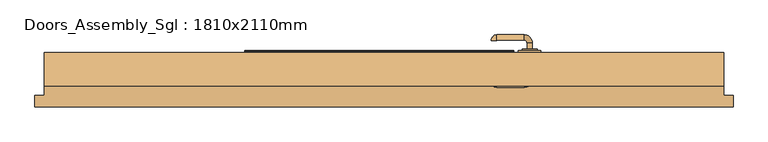
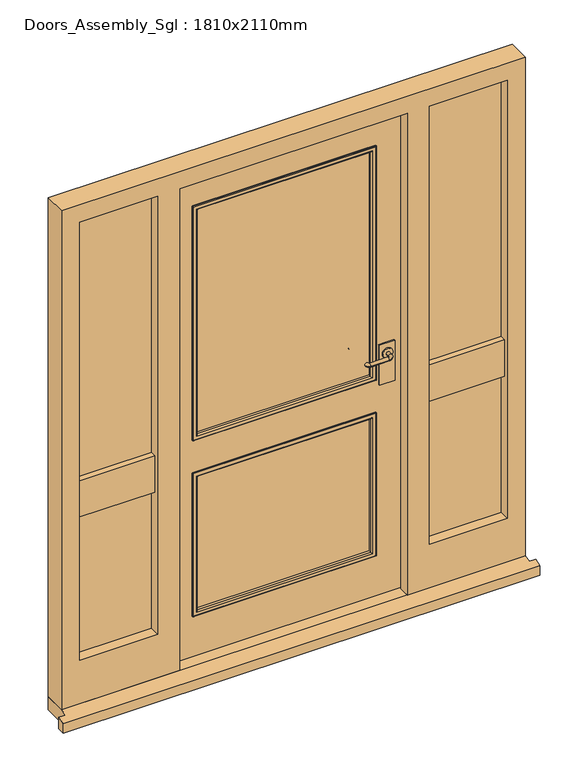
"""IFC4 building model written with IfcOpenShell, lengths in millimetres: door geometry, Doors_Assembly_Sgl : 1810x2110mm."""

from ifc_helpers import new_model, si_unit, point, frame, frame_2d, origin, place, context, project, spatial, polyline, circle_curve, ellipse_curve, trimmed, segment, composite_curve, outline, extrude, faceted_brep, source, transform, mapped, element, save
from ifc_brep_helpers import plane_surface, cylinder_surface, revolved_surface, advanced_brep


def doors_assembly_sgl_1810x2110mm_cdd653b2(model_context):
    return source(origin(), model_context, "Body", "SolidModel", [
        extrude(outline(composite_curve([segment(trimmed(circle_curve(frame_2d((1050.0, 680.0)), 20.0), [point((1050.0, 700.0))], [point((1050.0, 660.0))], False, "CARTESIAN"), True, "CONTINUOUS"), segment(trimmed(circle_curve(frame_2d((1050.0, 680.0)), 20.0), [point((1050.0, 660.0))], [point((1050.0, 700.0))], False, "CARTESIAN"), True, "CONTINUOUS")], self_intersect=False)), frame((0.0, -42.25, 0.0), z_axis=(0.0, 1.0, 0.0), x_axis=(0.0, 0.0, 1.0)), (0.0, 0.0, 1.0), 4.5929895),
        advanced_brep(
        [(673.0, -37.6570105, 1050.0), (687.0, -37.6570105, 1050.0), (687.0, -22.25, 1050.0), (673.0, -22.25, 1050.0), (665.0, -0.25, 1050.0), (665.0, -14.25, 1050.0), (593.0, -0.25, 1050.0), (593.0, -14.25, 1050.0), (592.0, -15.25, 1050.0), (578.0, -15.25, 1050.0)],
        [
            (0, 1, circle_curve(frame((680.0, -37.6570105, 1050.0), z_axis=(0.0, -1.0, 0.0), x_axis=(1.0, 0.0, 0.0)), 7.0)),
            (1, 0, circle_curve(frame((680.0, -37.6570105, 1050.0), z_axis=(0.0, -1.0, 0.0), x_axis=(1.0, 0.0, 0.0)), 7.0)),
            (1, 2),
            (2, 3, circle_curve(frame((680.0, -22.25, 1050.0), z_axis=(0.0, -1.0, 0.0), x_axis=(1.0, 0.0, 0.0)), 7.0)),
            (3, 0),
            (3, 2, circle_curve(frame((680.0, -22.25, 1050.0), z_axis=(0.0, -1.0, 0.0), x_axis=(1.0, 0.0, 0.0)), 7.0)),
            (4, 5, circle_curve(frame((665.0, -7.25, 1050.0), z_axis=(1.0, 0.0, 0.0), x_axis=(0.0, 1.0, 0.0)), 7.0)),
            (5, 3, circle_curve(frame((665.0, -22.25, 1050.0), z_axis=(0.0, 0.0, -1.0), x_axis=(1.0, 0.0, 0.0)), 8.0)),
            (2, 4, circle_curve(frame((665.0, -22.25, 1050.0), z_axis=(0.0, 0.0, 1.0), x_axis=(1.0, 0.0, 0.0)), 22.0)),
            (5, 4, circle_curve(frame((665.0, -7.25, 1050.0), z_axis=(1.0, 0.0, 0.0), x_axis=(0.0, 1.0, 0.0)), 7.0)),
            (4, 6),
            (6, 7, circle_curve(frame((593.0, -7.25, 1050.0), z_axis=(1.0, 0.0, 0.0), x_axis=(0.0, 1.0, 0.0)), 7.0)),
            (7, 5),
            (7, 6, circle_curve(frame((593.0, -7.25, 1050.0), z_axis=(1.0, 0.0, 0.0), x_axis=(0.0, 1.0, 0.0)), 7.0)),
            (8, 9, circle_curve(frame((585.0, -15.25, 1050.0), z_axis=(0.0, -1.0, 0.0), x_axis=(-1.0, 0.0, 0.0)), 7.0)),
            (9, 8, circle_curve(frame((585.0, -15.25, 1050.0), z_axis=(0.0, -1.0, 0.0), x_axis=(-1.0, 0.0, 0.0)), 7.0)),
            (8, 7, circle_curve(frame((593.0, -15.25, 1050.0), z_axis=(0.0, 0.0, -1.0), x_axis=(0.0, 1.0, 0.0)), 1.0)),
            (6, 9, circle_curve(frame((593.0, -15.25, 1050.0), z_axis=(0.0, 0.0, 1.0), x_axis=(0.0, 1.0, 0.0)), 15.0)),
        ],
        [
            plane_surface(frame((680.0, -37.6570105, 1050.0), z_axis=(0.0, -1.0, 0.0), x_axis=(0.0, 0.0, 1.0))),
            cylinder_surface(frame((680.0, -37.6570105, 1050.0), z_axis=(0.0, -1.0, 0.0), x_axis=(1.0, 0.0, 0.0)), 7.0),
            revolved_surface(trimmed(ellipse_curve(frame((680.0, -22.25, 1050.0), z_axis=(0.0, 1.0, 0.0), x_axis=(1.0, 0.0, 0.0)), 7.0, 7.0), [point((673.0, -22.25, 1050.0))], [point((687.0, -22.25, 1050.0))], True, "CARTESIAN"), (665.0, -22.25, 1050.0), (0.0, 0.0, -1.0)),
            revolved_surface(trimmed(ellipse_curve(frame((680.0, -22.25, 1050.0), z_axis=(0.0, 1.0, 0.0), x_axis=(1.0, 0.0, 0.0)), 7.0, 7.0), [point((687.0, -22.25, 1050.0))], [point((673.0, -22.25, 1050.0))], True, "CARTESIAN"), (665.0, -22.25, 1050.0), (0.0, 0.0, -1.0)),
            cylinder_surface(frame((665.0, -7.25, 1050.0), z_axis=(1.0, 0.0, 0.0), x_axis=(0.0, 1.0, 0.0)), 7.0),
            plane_surface(frame((585.0, -15.25, 1050.0), z_axis=(0.0, -1.0, 0.0), x_axis=(0.0, 0.0, 1.0))),
            revolved_surface(trimmed(ellipse_curve(frame((593.0, -7.25, 1050.0), z_axis=(-1.0, 0.0, 0.0), x_axis=(0.0, 1.0, 0.0)), 7.0, 7.0), [point((593.0, -14.25, 1050.0))], [point((593.0, -0.25, 1050.0))], True, "CARTESIAN"), (593.0, -15.25, 1050.0), (0.0, 0.0, -1.0)),
            revolved_surface(trimmed(ellipse_curve(frame((593.0, -7.25, 1050.0), z_axis=(-1.0, 0.0, 0.0), x_axis=(0.0, 1.0, 0.0)), 7.0, 7.0), [point((593.0, -0.25, 1050.0))], [point((593.0, -14.25, 1050.0))], True, "CARTESIAN"), (593.0, -15.25, 1050.0), (0.0, 0.0, -1.0)),
        ],
        [
            (0, [[1, 2]]),
            (1, [[3, 4, 5, -2]]),
            (1, [[-5, 6, -3, -1]]),
            (2, [[7, 8, -4, 9]]),
            (3, [[10, -9, -6, -8]]),
            (4, [[11, 12, 13, -7]]),
            (4, [[-13, 14, -11, -10]]),
            (5, [[15, 16]]),
            (6, [[-15, 17, -12, 18]]),
            (7, [[-16, -18, -14, -17]]),
        ],
    ),
        extrude(outline(polyline([(650.0, -48.25), (650.0, -42.25), (710.0, -42.25), (710.0, -48.25), (650.0, -48.25)])), frame((0.0, 0.0, 925.0), z_axis=(0.0, 0.0, 1.0), x_axis=(1.0, 0.0, 0.0)), (0.0, 0.0, 1.0), 165.0),
        extrude(outline(composite_curve([segment(trimmed(circle_curve(frame_2d((1050.0, 680.0)), 20.0), [point((1050.0, 700.0))], [point((1050.0, 660.0))], False, "CARTESIAN"), True, "CONTINUOUS"), segment(trimmed(circle_curve(frame_2d((1050.0, 680.0)), 20.0), [point((1050.0, 660.0))], [point((1050.0, 700.0))], False, "CARTESIAN"), True, "CONTINUOUS")], self_intersect=False)), frame((0.0, -102.8429895, 0.0), z_axis=(0.0, 1.0, 0.0), x_axis=(0.0, 0.0, 1.0)), (0.0, 0.0, 1.0), 4.5929895),
        advanced_brep(
        [(673.0, -102.8429895, 1050.0), (687.0, -102.8429895, 1050.0), (673.0, -118.25, 1050.0), (687.0, -118.25, 1050.0), (665.0, -140.25, 1050.0), (665.0, -126.25, 1050.0), (593.0, -126.25, 1050.0), (593.0, -140.25, 1050.0), (592.0, -125.25, 1050.0), (578.0, -125.25, 1050.0)],
        [
            (0, 1, circle_curve(frame((680.0, -102.8429895, 1050.0), z_axis=(0.0, 1.0, 0.0), x_axis=(1.0, 0.0, 0.0)), 7.0)),
            (1, 0, circle_curve(frame((680.0, -102.8429895, 1050.0), z_axis=(0.0, 1.0, 0.0), x_axis=(1.0, 0.0, 0.0)), 7.0)),
            (0, 2),
            (2, 3, circle_curve(frame((680.0, -118.25, 1050.0), z_axis=(0.0, 1.0, 0.0), x_axis=(1.0, 0.0, 0.0)), 7.0)),
            (3, 1),
            (3, 2, circle_curve(frame((680.0, -118.25, 1050.0), z_axis=(0.0, 1.0, 0.0), x_axis=(1.0, 0.0, 0.0)), 7.0)),
            (4, 3, circle_curve(frame((665.0, -118.25, 1050.0), z_axis=(0.0, 0.0, 1.0), x_axis=(1.0, 0.0, 0.0)), 22.0)),
            (2, 5, circle_curve(frame((665.0, -118.25, 1050.0), z_axis=(0.0, 0.0, -1.0), x_axis=(1.0, 0.0, 0.0)), 8.0)),
            (5, 4, circle_curve(frame((665.0, -133.25, 1050.0), z_axis=(1.0, 0.0, 0.0), x_axis=(0.0, -1.0, 0.0)), 7.0)),
            (4, 5, circle_curve(frame((665.0, -133.25, 1050.0), z_axis=(1.0, 0.0, 0.0), x_axis=(0.0, -1.0, 0.0)), 7.0)),
            (5, 6),
            (6, 7, circle_curve(frame((593.0, -133.25, 1050.0), z_axis=(1.0, 0.0, 0.0), x_axis=(0.0, -1.0, 0.0)), 7.0)),
            (7, 4),
            (7, 6, circle_curve(frame((593.0, -133.25, 1050.0), z_axis=(1.0, 0.0, 0.0), x_axis=(0.0, -1.0, 0.0)), 7.0)),
            (8, 9, circle_curve(frame((585.0, -125.25, 1050.0), z_axis=(0.0, 1.0, 0.0), x_axis=(-1.0, 0.0, 0.0)), 7.0)),
            (9, 8, circle_curve(frame((585.0, -125.25, 1050.0), z_axis=(0.0, 1.0, 0.0), x_axis=(-1.0, 0.0, 0.0)), 7.0)),
            (9, 7, circle_curve(frame((593.0, -125.25, 1050.0), z_axis=(0.0, 0.0, 1.0), x_axis=(0.0, -1.0, 0.0)), 15.0)),
            (6, 8, circle_curve(frame((593.0, -125.25, 1050.0), z_axis=(0.0, 0.0, -1.0), x_axis=(0.0, -1.0, 0.0)), 1.0)),
        ],
        [
            plane_surface(frame((680.0, -102.8429895, 1050.0), z_axis=(0.0, 1.0, 0.0), x_axis=(0.0, 0.0, 1.0))),
            cylinder_surface(frame((680.0, -102.8429895, 1050.0), z_axis=(0.0, 1.0, 0.0), x_axis=(1.0, 0.0, 0.0)), 7.0),
            revolved_surface(trimmed(ellipse_curve(frame((680.0, -118.25, 1050.0), z_axis=(0.0, 1.0, 0.0), x_axis=(1.0, 0.0, 0.0)), 7.0, 7.0), [point((673.0, -118.25, 1050.0))], [point((687.0, -118.25, 1050.0))], True, "CARTESIAN"), (665.0, -118.25, 1050.0), (0.0, 0.0, -1.0)),
            revolved_surface(trimmed(ellipse_curve(frame((680.0, -118.25, 1050.0), z_axis=(0.0, 1.0, 0.0), x_axis=(1.0, 0.0, 0.0)), 7.0, 7.0), [point((687.0, -118.25, 1050.0))], [point((673.0, -118.25, 1050.0))], True, "CARTESIAN"), (665.0, -118.25, 1050.0), (0.0, 0.0, -1.0)),
            cylinder_surface(frame((665.0, -133.25, 1050.0), z_axis=(1.0, 0.0, 0.0), x_axis=(0.0, -1.0, 0.0)), 7.0),
            plane_surface(frame((585.0, -125.25, 1050.0), z_axis=(0.0, 1.0, 0.0), x_axis=(0.0, 0.0, 1.0))),
            revolved_surface(trimmed(ellipse_curve(frame((593.0, -133.25, 1050.0), z_axis=(1.0, 0.0, 0.0), x_axis=(0.0, -1.0, 0.0)), 7.0, 7.0), [point((593.0, -126.25, 1050.0))], [point((593.0, -140.25, 1050.0))], True, "CARTESIAN"), (593.0, -125.25, 1050.0), (0.0, 0.0, -1.0)),
            revolved_surface(trimmed(ellipse_curve(frame((593.0, -133.25, 1050.0), z_axis=(1.0, 0.0, 0.0), x_axis=(0.0, -1.0, 0.0)), 7.0, 7.0), [point((593.0, -140.25, 1050.0))], [point((593.0, -126.25, 1050.0))], True, "CARTESIAN"), (593.0, -125.25, 1050.0), (0.0, 0.0, -1.0)),
        ],
        [
            (0, [[1, 2]]),
            (1, [[-1, 3, 4, 5]]),
            (1, [[-2, -5, 6, -3]]),
            (2, [[7, -4, 8, 9]]),
            (3, [[-8, -6, -7, 10]]),
            (4, [[-9, 11, 12, 13]]),
            (4, [[-10, -13, 14, -11]]),
            (5, [[15, 16]]),
            (6, [[17, -12, 18, -16]]),
            (7, [[-18, -14, -17, -15]]),
        ],
    ),
        extrude(outline(polyline([(650.0, -92.25), (710.0, -92.25), (710.0, -98.25), (650.0, -98.25), (650.0, -92.25)])), frame((0.0, 0.0, 925.0), z_axis=(0.0, 0.0, 1.0), x_axis=(1.0, 0.0, 0.0)), (0.0, 0.0, 1.0), 165.0),
        extrude(outline(polyline([(1148.5, -71.25), (1148.5, -95.25), (800.0, -95.25), (800.0, -71.25), (1148.5, -71.25)])), frame((0.0, 0.0, 218.5), z_axis=(0.0, 0.0, 1.0), x_axis=(1.0, 0.0, 0.0)), (0.0, 0.0, 1.0), 605.0),
        extrude(outline(polyline([(1148.5, -71.25), (1148.5, -95.25), (800.0, -95.25), (800.0, -71.25), (1148.5, -71.25)])), frame((0.0, 0.0, 943.5), z_axis=(0.0, 0.0, 1.0), x_axis=(1.0, 0.0, 0.0)), (0.0, 0.0, 1.0), 1118.0),
        extrude(outline(polyline([(-216.0, -71.25), (-216.0, -95.25), (-564.5, -95.25), (-564.5, -71.25), (-216.0, -71.25)])), frame((0.0, 0.0, 218.5), z_axis=(0.0, 0.0, 1.0), x_axis=(1.0, 0.0, 0.0)), (0.0, 0.0, 1.0), 605.0),
        extrude(outline(polyline([(-216.0, -71.25), (-216.0, -95.25), (-564.5, -95.25), (-564.5, -71.25), (-216.0, -71.25)])), frame((0.0, 0.0, 943.5), z_axis=(0.0, 0.0, 1.0), x_axis=(1.0, 0.0, 0.0)), (0.0, 0.0, 1.0), 1118.0),
        faceted_brep([(1197.0, -137.25, 54.5), (736.0, -137.25, 54.5), (736.0, -95.25, 54.5), (758.0, -95.25, 54.5), (758.0, -48.25, 54.5), (1197.0, -48.25, 54.5), (1197.0, -48.25, 2110.0), (1197.0, -137.25, 2110.0), (758.0, -48.25, 2061.5), (-174.0, -48.25, 2061.5), (-174.0, -48.25, 54.5), (-613.0, -48.25, 54.5), (-613.0, -48.25, 2110.0), (1126.5, -48.25, 958.5), (1126.5, -48.25, 2039.5), (822.0, -48.25, 2039.5), (822.0, -48.25, 958.5), (822.0, -48.25, 808.5), (822.0, -48.25, 233.5), (1126.5, -48.25, 233.5), (1126.5, -48.25, 808.5), (-238.0, -48.25, 808.5), (-542.5, -48.25, 808.5), (-542.5, -48.25, 233.5), (-238.0, -48.25, 233.5), (-542.5, -48.25, 2039.5), (-542.5, -48.25, 958.5), (-238.0, -48.25, 958.5), (-238.0, -48.25, 2039.5), (758.0, -95.25, 2061.5), (-174.0, -95.25, 54.5), (-174.0, -95.25, 2061.5), (736.0, -95.25, 2039.5), (-152.0, -95.25, 2039.5), (-152.0, -95.25, 54.5), (-216.0, -95.25, 2061.5), (-216.0, -95.25, 943.5), (-564.5, -95.25, 943.5), (-564.5, -95.25, 2061.5), (-542.5, -95.25, 2039.5), (-542.5, -95.25, 958.5), (-238.0, -95.25, 958.5), (-238.0, -95.25, 2039.5), (1148.5, -95.25, 2061.5), (1148.5, -95.25, 943.5), (800.0, -95.25, 943.5), (800.0, -95.25, 2061.5), (822.0, -95.25, 2039.5), (822.0, -95.25, 958.5), (1126.5, -95.25, 958.5), (1126.5, -95.25, 2039.5), (1148.5, -95.25, 218.5), (800.0, -95.25, 218.5), (800.0, -95.25, 823.5), (1148.5, -95.25, 823.5), (1126.5, -95.25, 808.5), (822.0, -95.25, 808.5), (822.0, -95.25, 233.5), (1126.5, -95.25, 233.5), (-564.5, -95.25, 823.5), (-216.0, -95.25, 823.5), (-216.0, -95.25, 218.5), (-564.5, -95.25, 218.5), (-238.0, -95.25, 808.5), (-542.5, -95.25, 808.5), (-542.5, -95.25, 233.5), (-238.0, -95.25, 233.5), (736.0, -137.25, 2039.5), (-613.0, -137.25, 54.5), (-152.0, -137.25, 54.5), (-152.0, -137.25, 2039.5), (-613.0, -137.25, 2110.0), (-238.0, -137.25, 2039.5), (-238.0, -137.25, 233.5), (-542.5, -137.25, 233.5), (-542.5, -137.25, 2039.5), (1126.5, -137.25, 2039.5), (1126.5, -137.25, 233.5), (822.0, -137.25, 233.5), (822.0, -137.25, 2039.5), (-542.5, -118.25, 808.5), (-542.5, -118.25, 958.5), (-238.0, -118.25, 958.5), (-238.0, -118.25, 808.5), (822.0, -118.25, 808.5), (822.0, -118.25, 958.5), (1126.5, -118.25, 958.5), (1126.5, -118.25, 808.5), (822.0, -71.25, 958.5), (1126.5, -71.25, 958.5), (822.0, -71.25, 2039.5), (822.0, -71.25, 808.5), (822.0, -71.25, 233.5), (1126.5, -71.25, 2039.5), (1126.5, -71.25, 233.5), (1126.5, -71.25, 808.5), (-238.0, -71.25, 958.5), (-238.0, -71.25, 2039.5), (-238.0, -71.25, 233.5), (-238.0, -71.25, 808.5), (-542.5, -71.25, 233.5), (-542.5, -71.25, 2039.5), (-542.5, -71.25, 958.5), (-542.5, -71.25, 808.5), (1148.5, -71.25, 218.5), (1148.5, -71.25, 823.5), (1148.5, -71.25, 943.5), (1148.5, -71.25, 2061.5), (800.0, -71.25, 823.5), (800.0, -71.25, 218.5), (800.0, -71.25, 2061.5), (800.0, -71.25, 943.5), (-564.5, -71.25, 218.5), (-564.5, -71.25, 823.5), (-564.5, -71.25, 943.5), (-564.5, -71.25, 2061.5), (-216.0, -71.25, 943.5), (-216.0, -71.25, 2061.5), (-216.0, -71.25, 823.5), (-216.0, -71.25, 218.5)], [[[0, 1, 2, 3, 4, 5]], [[5, 6, 7, 0]], [[5, 4, 8, 9, 10, 11, 12, 6], [13, 14, 15, 16], [17, 18, 19, 20], [21, 22, 23, 24], [25, 26, 27, 28]], [[3, 29, 8, 4]], [[30, 31, 29, 3, 2, 32, 33, 34]], [[35, 36, 37, 38], [39, 40, 41, 42]], [[43, 44, 45, 46], [47, 48, 49, 50]], [[51, 52, 53, 54], [55, 56, 57, 58]], [[59, 60, 61, 62], [63, 64, 65, 66]], [[1, 67, 32, 2]], [[68, 69, 70, 67, 1, 0, 7, 71], [72, 73, 74, 75], [76, 77, 78, 79]], [[71, 12, 11, 68]], [[34, 33, 70, 69]], [[11, 10, 30, 34, 69, 68]], [[75, 74, 65, 64, 80, 81, 40, 39]], [[65, 74, 73, 66]], [[42, 41, 82, 83, 63, 66, 73, 72]], [[79, 78, 57, 56, 84, 85, 48, 47]], [[77, 58, 57, 78]], [[50, 49, 86, 87, 55, 58, 77, 76]], [[16, 88, 89, 13]], [[90, 88, 16, 15]], [[17, 91, 92, 18]], [[14, 13, 89, 93]], [[19, 94, 95, 20]], [[20, 95, 91, 17]], [[18, 92, 94, 19]], [[28, 27, 96, 97]], [[24, 98, 99, 21]], [[23, 100, 98, 24]], [[101, 102, 26, 25]], [[22, 103, 100, 23]], [[21, 99, 103, 22]], [[26, 102, 96, 27]], [[10, 9, 31, 30]], [[104, 51, 54, 105]], [[106, 44, 43, 107]], [[104, 105, 108, 109], [94, 92, 91, 95]], [[110, 111, 106, 107], [93, 89, 88, 90]], [[54, 53, 108, 105]], [[109, 52, 51, 104]], [[111, 45, 44, 106]], [[40, 81, 82, 41]], [[112, 113, 59, 62]], [[114, 115, 38, 37]], [[37, 36, 116, 114]], [[36, 35, 117, 116]], [[61, 60, 118, 119]], [[48, 85, 86, 49]], [[108, 53, 52, 109]], [[110, 46, 45, 111]], [[55, 87, 84, 56]], [[63, 83, 80, 64]], [[112, 62, 61, 119]], [[113, 118, 60, 59]], [[85, 84, 87, 86]], [[115, 114, 116, 117], [97, 96, 102, 101]], [[119, 118, 113, 112], [100, 103, 99, 98]], [[81, 80, 83, 82]], [[7, 6, 12, 71]], [[9, 8, 29, 31]], [[38, 115, 117, 35]], [[46, 110, 107, 43]], [[76, 79, 47, 50]], [[33, 32, 67, 70]], [[39, 42, 72, 75]], [[101, 25, 28, 97]], [[14, 93, 90, 15]]]),
        extrude(outline(polyline([(-71.0, -82.25), (-71.0, -58.25), (630.0, -58.25), (630.0, -82.25), (-71.0, -82.25)])), frame((0.0, 0.0, 958.5), z_axis=(0.0, 0.0, 1.0), x_axis=(1.0, 0.0, 0.0)), (0.0, 0.0, 1.0), 950.0),
        extrude(outline(polyline([(-71.0, -82.25), (-71.0, -58.25), (630.0, -58.25), (630.0, -82.25), (-71.0, -82.25)])), frame((0.0, 0.0, 233.5), z_axis=(0.0, 0.0, 1.0), x_axis=(1.0, 0.0, 0.0)), (0.0, 0.0, 1.0), 575.0),
        faceted_brep([(1222.0, -192.25, 0.0), (1222.0, -162.25, 0.0), (1222.0, -162.25, 47.2703282), (1222.0, -192.25, 38.5947221), (-638.0, -192.25, 38.5947221), (-638.0, -162.25, 47.2703282), (-638.0, -162.25, 0.0), (-638.0, -192.25, 0.0), (-613.0, -162.25, 0.0), (-613.0, -48.25, 0.0), (1197.0, -48.25, 0.0), (1197.0, -162.25, 0.0), (1197.0, -162.25, 47.2703282), (1197.0, -137.25, 54.5), (-613.0, -137.25, 54.5), (-613.0, -162.25, 47.2703282), (1197.0, -48.25, 54.5), (-613.0, -48.25, 54.5)], [[[0, 1, 2, 3]], [[4, 5, 6, 7]], [[7, 6, 8, 9, 10, 11, 1, 0]], [[3, 4, 7, 0]], [[3, 2, 12, 13, 14, 15, 5, 4]], [[14, 13, 16, 17]], [[17, 16, 10, 9]], [[15, 14, 17, 9, 8]], [[8, 6, 5, 15]], [[11, 10, 16, 13, 12]], [[12, 2, 1, 11]]]),
        extrude(outline(polyline([(58.5, -171.0), (58.5, 755.0), (2058.5, 755.0), (2058.5, -171.0), (58.5, -171.0)]), holes=[polyline([(1908.5, 630.0), (958.5, 630.0), (958.5, -71.0), (1908.5, -71.0), (1908.5, 630.0)]), polyline([(808.5, -71.0), (808.5, 630.0), (233.5, 630.0), (233.5, -71.0), (808.5, -71.0)])]), frame((0.0, -92.25, 0.0), z_axis=(0.0, 1.0, 0.0), x_axis=(0.0, 0.0, 1.0)), (0.0, 0.0, 1.0), 44.0),
        advanced_brep(
        [(630.0, -58.25, 808.5), (630.0, -58.25, 233.5), (630.0, -48.25, 233.5), (630.0, -48.25, 808.5), (618.0, -47.25, 796.5), (618.0, -47.25, 245.5), (618.0, -58.25, 245.5), (618.0, -58.25, 796.5), (623.0, -42.25, 801.5), (623.0, -42.25, 240.5), (638.0, -44.25, 816.5), (638.0, -44.25, 225.5), (636.0, -42.25, 227.5), (636.0, -42.25, 814.5), (638.0, -48.25, 816.5), (638.0, -48.25, 225.5), (-71.0, -58.25, 233.5), (-71.0, -48.25, 233.5), (-59.0, -47.25, 245.5), (-59.0, -58.25, 245.5), (-64.0, -42.25, 240.5), (-79.0, -44.25, 225.5), (-77.0, -42.25, 227.5), (-79.0, -48.25, 225.5), (-71.0, -58.25, 808.5), (-71.0, -48.25, 808.5), (-59.0, -47.25, 796.5), (-59.0, -58.25, 796.5), (-64.0, -42.25, 801.5), (-79.0, -44.25, 816.5), (-77.0, -42.25, 814.5), (-79.0, -48.25, 816.5)],
        [
            (0, 1),
            (1, 2),
            (2, 3),
            (3, 0),
            (4, 5),
            (5, 6),
            (6, 7),
            (7, 4),
            (8, 9),
            (9, 5, ellipse_curve(frame((623.0, -47.25, 240.5), z_axis=(0.7071067811865429, 0.0, 0.707106781186552), x_axis=(-0.7071067811865519, 0.0, 0.7071067811865431)), 7.0710678, 5.0)),
            (4, 8, ellipse_curve(frame((623.0, -47.25, 801.5), z_axis=(0.707106781186552, 0.0, -0.707106781186543), x_axis=(0.7071067811865429, 0.0, 0.707106781186552)), 7.0710678, 5.0)),
            (10, 11),
            (11, 12, ellipse_curve(frame((636.0, -44.25, 227.5), z_axis=(0.7071067811865429, 0.0, 0.707106781186552), x_axis=(-0.7071067811865519, 0.0, 0.7071067811865431)), 2.8284271, 2.0)),
            (12, 13),
            (13, 10, ellipse_curve(frame((636.0, -44.25, 814.5), z_axis=(0.707106781186552, 0.0, -0.707106781186543), x_axis=(0.7071067811865429, 0.0, 0.707106781186552)), 2.8284271, 2.0)),
            (14, 15),
            (15, 11),
            (10, 14),
            (1, 16),
            (16, 17),
            (17, 2),
            (5, 18),
            (18, 19),
            (19, 6),
            (9, 20),
            (20, 18, ellipse_curve(frame((-64.0, -47.25, 240.5), z_axis=(0.707106781186552, 0.0, -0.7071067811865431), x_axis=(0.7071067811865429, 0.0, 0.707106781186552)), 7.0710678, 5.0)),
            (11, 21),
            (21, 22, ellipse_curve(frame((-77.0, -44.25, 227.5), z_axis=(0.707106781186552, 0.0, -0.7071067811865431), x_axis=(0.7071067811865429, 0.0, 0.707106781186552)), 2.8284271, 2.0)),
            (22, 12),
            (15, 23),
            (23, 21),
            (16, 24),
            (24, 25),
            (25, 17),
            (18, 26),
            (26, 27),
            (27, 19),
            (20, 28),
            (28, 26, ellipse_curve(frame((-64.0, -47.25, 801.5), z_axis=(-0.707106781186543, 0.0, -0.7071067811865519), x_axis=(0.7071067811865518, 0.0, -0.7071067811865431)), 7.0710678, 5.0)),
            (21, 29),
            (29, 30, ellipse_curve(frame((-77.0, -44.25, 814.5), z_axis=(-0.707106781186543, 0.0, -0.7071067811865519), x_axis=(0.7071067811865518, 0.0, -0.7071067811865431)), 2.8284271, 2.0)),
            (30, 22),
            (23, 31),
            (31, 29),
            (14, 31),
            (25, 3),
            (24, 0),
            (27, 7),
            (26, 4),
            (28, 8),
            (30, 13),
            (29, 10),
        ],
        [
            plane_surface(frame((630.0, -48.25, 808.5), z_axis=(1.0, 0.0, 0.0), x_axis=(0.0, 0.0, -1.0))),
            plane_surface(frame((618.0, -58.25, 796.5), z_axis=(-1.0, 0.0, 0.0), x_axis=(0.0, 0.0, -1.0))),
            cylinder_surface(frame((623.0, -47.25, 808.5), z_axis=(0.0, 0.0, 1.0), x_axis=(1.0, 0.0, 0.0)), 5.0),
            cylinder_surface(frame((636.0, -44.25, 808.5), z_axis=(0.0, 0.0, 1.0), x_axis=(1.0, 0.0, 0.0)), 2.0),
            plane_surface(frame((638.0, -44.25, 816.5), z_axis=(1.0, 0.0, 0.0), x_axis=(0.0, 0.0, -1.0))),
            plane_surface(frame((630.0, -48.25, 233.5), z_axis=(0.0, 0.0, -1.0), x_axis=(-1.0, 0.0, 0.0))),
            plane_surface(frame((618.0, -58.25, 245.5), z_axis=(0.0, 0.0, 1.0), x_axis=(-1.0, 0.0, 0.0))),
            cylinder_surface(frame((630.0, -47.25, 240.5), z_axis=(1.0, 0.0, 0.0), x_axis=(0.0, 0.0, -1.0)), 5.0),
            cylinder_surface(frame((630.0, -44.25, 227.5), z_axis=(1.0, 0.0, 0.0), x_axis=(0.0, 0.0, -1.0)), 2.0),
            plane_surface(frame((638.0, -44.25, 225.5), z_axis=(0.0, 0.0, -1.0), x_axis=(-1.0, 0.0, 0.0))),
            plane_surface(frame((-71.0, -48.25, 233.5), z_axis=(-1.0, 0.0, 0.0), x_axis=(0.0, 0.0, 1.0))),
            plane_surface(frame((-59.0, -58.25, 245.5), z_axis=(1.0, 0.0, 0.0), x_axis=(0.0, 0.0, 1.0))),
            cylinder_surface(frame((-64.0, -47.25, 233.5), z_axis=(0.0, 0.0, -1.0), x_axis=(-1.0, 0.0, 0.0)), 5.0),
            cylinder_surface(frame((-77.0, -44.25, 233.5), z_axis=(0.0, 0.0, -1.0), x_axis=(-1.0, 0.0, 0.0)), 2.0),
            plane_surface(frame((-79.0, -44.25, 225.5), z_axis=(-1.0, 0.0, 0.0), x_axis=(0.0, 0.0, 1.0))),
            plane_surface(frame((-79.0, -48.25, 816.5), z_axis=(0.0, -1.0, 0.0), x_axis=(1.0, 0.0, 0.0))),
            plane_surface(frame((-71.0, -48.25, 808.5), z_axis=(0.0, 0.0, 1.0), x_axis=(1.0, 0.0, 0.0))),
            plane_surface(frame((-71.0, -58.25, 808.5), z_axis=(0.0, -1.0, 0.0), x_axis=(1.0, 0.0, 0.0))),
            plane_surface(frame((-59.0, -58.25, 796.5), z_axis=(0.0, 0.0, -1.0), x_axis=(1.0, 0.0, 0.0))),
            cylinder_surface(frame((-71.0, -47.25, 801.5), z_axis=(-1.0, 0.0, 0.0), x_axis=(0.0, 0.0, 1.0)), 5.0),
            plane_surface(frame((-64.0, -42.25, 801.5), z_axis=(0.0, 1.0, 0.0), x_axis=(1.0, 0.0, 0.0))),
            cylinder_surface(frame((-71.0, -44.25, 814.5), z_axis=(-1.0, 0.0, 0.0), x_axis=(0.0, 0.0, 1.0)), 2.0),
            plane_surface(frame((-79.0, -44.25, 816.5), z_axis=(0.0, 0.0, 1.0), x_axis=(1.0, 0.0, 0.0))),
        ],
        [
            (0, [[1, 2, 3, 4]]),
            (1, [[5, 6, 7, 8]]),
            (2, [[9, 10, -5, 11]]),
            (3, [[12, 13, 14, 15]]),
            (4, [[16, 17, -12, 18]]),
            (5, [[19, 20, 21, -2]]),
            (6, [[22, 23, 24, -6]]),
            (7, [[25, 26, -22, -10]]),
            (8, [[27, 28, 29, -13]]),
            (9, [[30, 31, -27, -17]]),
            (10, [[32, 33, 34, -20]]),
            (11, [[35, 36, 37, -23]]),
            (12, [[38, 39, -35, -26]]),
            (13, [[40, 41, 42, -28]]),
            (14, [[43, 44, -40, -31]]),
            (15, [[-16, 45, -43, -30], [-3, -21, -34, 46]]),
            (16, [[47, -4, -46, -33]]),
            (17, [[-1, -47, -32, -19], [-7, -24, -37, 48]]),
            (18, [[49, -8, -48, -36]]),
            (19, [[50, -11, -49, -39]]),
            (20, [[-14, -29, -42, 51], [-9, -50, -38, -25]]),
            (21, [[52, -15, -51, -41]]),
            (22, [[-45, -18, -52, -44]]),
        ],
    ),
        advanced_brep(
        [(-71.0, -82.25, 808.5), (-71.0, -82.25, 233.5), (-71.0, -92.25, 233.5), (-71.0, -92.25, 808.5), (-59.0, -93.25, 796.5), (-59.0, -93.25, 245.5), (-59.0, -82.25, 245.5), (-59.0, -82.25, 796.5), (-64.0, -98.25, 801.5), (-64.0, -98.25, 240.5), (-79.0, -96.25, 816.5), (-79.0, -96.25, 225.5), (-77.0, -98.25, 227.5), (-77.0, -98.25, 814.5), (-79.0, -92.25, 816.5), (-79.0, -92.25, 225.5), (630.0, -82.25, 233.5), (630.0, -92.25, 233.5), (618.0, -93.25, 245.5), (618.0, -82.25, 245.5), (623.0, -98.25, 240.5), (638.0, -96.25, 225.5), (636.0, -98.25, 227.5), (638.0, -92.25, 225.5), (630.0, -82.25, 808.5), (630.0, -92.25, 808.5), (618.0, -93.25, 796.5), (618.0, -82.25, 796.5), (623.0, -98.25, 801.5), (638.0, -96.25, 816.5), (636.0, -98.25, 814.5), (638.0, -92.25, 816.5)],
        [
            (0, 1),
            (1, 2),
            (2, 3),
            (3, 0),
            (4, 5),
            (5, 6),
            (6, 7),
            (7, 4),
            (8, 9),
            (9, 5, ellipse_curve(frame((-64.0, -93.25, 240.5), z_axis=(-0.7071067811865475, 0.0, 0.7071067811865475), x_axis=(0.7071067811865474, 0.0, 0.7071067811865476)), 7.0710678, 5.0)),
            (4, 8, ellipse_curve(frame((-64.0, -93.25, 801.5), z_axis=(-0.7071067811865475, 0.0, -0.7071067811865475), x_axis=(-0.7071067811865474, 0.0, 0.7071067811865477)), 7.0710678, 5.0)),
            (10, 11),
            (11, 12, ellipse_curve(frame((-77.0, -96.25, 227.5), z_axis=(-0.7071067811865475, 0.0, 0.7071067811865475), x_axis=(0.7071067811865474, 0.0, 0.7071067811865476)), 2.8284271, 2.0)),
            (12, 13),
            (13, 10, ellipse_curve(frame((-77.0, -96.25, 814.5), z_axis=(-0.7071067811865475, 0.0, -0.7071067811865475), x_axis=(-0.7071067811865474, 0.0, 0.7071067811865477)), 2.8284271, 2.0)),
            (14, 15),
            (15, 11),
            (10, 14),
            (1, 16),
            (16, 17),
            (17, 2),
            (5, 18),
            (18, 19),
            (19, 6),
            (9, 20),
            (20, 18, ellipse_curve(frame((623.0, -93.25, 240.5), z_axis=(-0.7071067811865475, 0.0, -0.7071067811865475), x_axis=(-0.7071067811865476, 0.0, 0.7071067811865474)), 7.0710678, 5.0)),
            (11, 21),
            (21, 22, ellipse_curve(frame((636.0, -96.25, 227.5), z_axis=(-0.7071067811865475, 0.0, -0.7071067811865475), x_axis=(-0.7071067811865476, 0.0, 0.7071067811865474)), 2.8284271, 2.0)),
            (22, 12),
            (15, 23),
            (23, 21),
            (16, 24),
            (24, 25),
            (25, 17),
            (18, 26),
            (26, 27),
            (27, 19),
            (20, 28),
            (28, 26, ellipse_curve(frame((623.0, -93.25, 801.5), z_axis=(0.7071067811865475, 0.0, -0.7071067811865475), x_axis=(-0.7071067811865474, 0.0, -0.7071067811865477)), 7.0710678, 5.0)),
            (21, 29),
            (29, 30, ellipse_curve(frame((636.0, -96.25, 814.5), z_axis=(0.7071067811865475, 0.0, -0.7071067811865475), x_axis=(-0.7071067811865474, 0.0, -0.7071067811865477)), 2.8284271, 2.0)),
            (30, 22),
            (23, 31),
            (31, 29),
            (14, 31),
            (25, 3),
            (24, 0),
            (27, 7),
            (26, 4),
            (28, 8),
            (30, 13),
            (29, 10),
        ],
        [
            plane_surface(frame((-71.0, -92.25, 808.5), z_axis=(-1.0, 0.0, 0.0), x_axis=(0.0, 0.0, -1.0))),
            plane_surface(frame((-59.0, -82.25, 796.5), z_axis=(1.0, 0.0, 0.0), x_axis=(0.0, 0.0, -1.0))),
            cylinder_surface(frame((-64.0, -93.25, 808.5), z_axis=(0.0, 0.0, 1.0), x_axis=(-1.0, 0.0, 0.0)), 5.0),
            cylinder_surface(frame((-77.0, -96.25, 808.5), z_axis=(0.0, 0.0, 1.0), x_axis=(-1.0, 0.0, 0.0)), 2.0),
            plane_surface(frame((-79.0, -96.25, 816.5), z_axis=(-1.0, 0.0, 0.0), x_axis=(0.0, 0.0, -1.0))),
            plane_surface(frame((-71.0, -92.25, 233.5), z_axis=(0.0, 0.0, -1.0), x_axis=(1.0, 0.0, 0.0))),
            plane_surface(frame((-59.0, -82.25, 245.5), z_axis=(0.0, 0.0, 1.0), x_axis=(1.0, 0.0, 0.0))),
            cylinder_surface(frame((-71.0, -93.25, 240.5), z_axis=(-1.0, 0.0, 0.0), x_axis=(0.0, 0.0, -1.0)), 5.0),
            cylinder_surface(frame((-71.0, -96.25, 227.5), z_axis=(-1.0, 0.0, 0.0), x_axis=(0.0, 0.0, -1.0)), 2.0),
            plane_surface(frame((-79.0, -96.25, 225.5), z_axis=(0.0, 0.0, -1.0), x_axis=(1.0, 0.0, 0.0))),
            plane_surface(frame((630.0, -92.25, 233.5), z_axis=(1.0, 0.0, 0.0), x_axis=(0.0, 0.0, 1.0))),
            plane_surface(frame((618.0, -82.25, 245.5), z_axis=(-1.0, 0.0, 0.0), x_axis=(0.0, 0.0, 1.0))),
            cylinder_surface(frame((623.0, -93.25, 233.5), z_axis=(0.0, 0.0, -1.0), x_axis=(1.0, 0.0, 0.0)), 5.0),
            cylinder_surface(frame((636.0, -96.25, 233.5), z_axis=(0.0, 0.0, -1.0), x_axis=(1.0, 0.0, 0.0)), 2.0),
            plane_surface(frame((638.0, -96.25, 225.5), z_axis=(1.0, 0.0, 0.0), x_axis=(0.0, 0.0, 1.0))),
            plane_surface(frame((638.0, -92.25, 816.5), z_axis=(0.0, 1.0, 0.0), x_axis=(-1.0, 0.0, 0.0))),
            plane_surface(frame((630.0, -92.25, 808.5), z_axis=(0.0, 0.0, 1.0), x_axis=(-1.0, 0.0, 0.0))),
            plane_surface(frame((630.0, -82.25, 808.5), z_axis=(0.0, 1.0, 0.0), x_axis=(-1.0, 0.0, 0.0))),
            plane_surface(frame((618.0, -82.25, 796.5), z_axis=(0.0, 0.0, -1.0), x_axis=(-1.0, 0.0, 0.0))),
            cylinder_surface(frame((630.0, -93.25, 801.5), z_axis=(1.0, 0.0, 0.0), x_axis=(0.0, 0.0, 1.0)), 5.0),
            plane_surface(frame((623.0, -98.25, 801.5), z_axis=(0.0, -1.0, 0.0), x_axis=(-1.0, 0.0, 0.0))),
            cylinder_surface(frame((630.0, -96.25, 814.5), z_axis=(1.0, 0.0, 0.0), x_axis=(0.0, 0.0, 1.0)), 2.0),
            plane_surface(frame((638.0, -96.25, 816.5), z_axis=(0.0, 0.0, 1.0), x_axis=(-1.0, 0.0, 0.0))),
        ],
        [
            (0, [[1, 2, 3, 4]]),
            (1, [[5, 6, 7, 8]]),
            (2, [[9, 10, -5, 11]]),
            (3, [[12, 13, 14, 15]]),
            (4, [[16, 17, -12, 18]]),
            (5, [[19, 20, 21, -2]]),
            (6, [[22, 23, 24, -6]]),
            (7, [[25, 26, -22, -10]]),
            (8, [[27, 28, 29, -13]]),
            (9, [[30, 31, -27, -17]]),
            (10, [[32, 33, 34, -20]]),
            (11, [[35, 36, 37, -23]]),
            (12, [[38, 39, -35, -26]]),
            (13, [[40, 41, 42, -28]]),
            (14, [[43, 44, -40, -31]]),
            (15, [[-16, 45, -43, -30], [-3, -21, -34, 46]]),
            (16, [[47, -4, -46, -33]]),
            (17, [[-1, -47, -32, -19], [-7, -24, -37, 48]]),
            (18, [[49, -8, -48, -36]]),
            (19, [[50, -11, -49, -39]]),
            (20, [[-14, -29, -42, 51], [-9, -50, -38, -25]]),
            (21, [[52, -15, -51, -41]]),
            (22, [[-45, -18, -52, -44]]),
        ],
    ),
        advanced_brep(
        [(-79.0, -96.25, 950.5), (-79.0, -96.25, 1916.5), (-79.0, -92.25, 1916.5), (-79.0, -92.25, 950.5), (-77.0, -98.25, 952.5), (-77.0, -98.25, 1914.5), (-59.0, -93.25, 970.5), (-59.0, -93.25, 1896.5), (-64.0, -98.25, 1901.5), (-64.0, -98.25, 965.5), (-59.0, -82.25, 970.5), (-59.0, -82.25, 1896.5), (-71.0, -92.25, 958.5), (-71.0, -92.25, 1908.5), (-71.0, -82.25, 1908.5), (-71.0, -82.25, 958.5), (638.0, -96.25, 1916.5), (638.0, -92.25, 1916.5), (636.0, -98.25, 1914.5), (618.0, -93.25, 1896.5), (623.0, -98.25, 1901.5), (618.0, -82.25, 1896.5), (630.0, -92.25, 1908.5), (630.0, -82.25, 1908.5), (638.0, -96.25, 950.5), (638.0, -92.25, 950.5), (636.0, -98.25, 952.5), (618.0, -93.25, 970.5), (623.0, -98.25, 965.5), (618.0, -82.25, 970.5), (630.0, -92.25, 958.5), (630.0, -82.25, 958.5)],
        [
            (0, 1),
            (1, 2),
            (2, 3),
            (3, 0),
            (4, 5),
            (5, 1, ellipse_curve(frame((-77.0, -96.25, 1914.5), z_axis=(-0.7071067811865476, 0.0, -0.7071067811865474), x_axis=(0.7071067811865472, 0.0, -0.7071067811865478)), 2.8284271, 2.0)),
            (0, 4, ellipse_curve(frame((-77.0, -96.25, 952.5), z_axis=(-0.7071067811865474, 0.0, 0.7071067811865476), x_axis=(-0.7071067811865475, 0.0, -0.7071067811865475)), 2.8284271, 2.0)),
            (6, 7),
            (7, 8, ellipse_curve(frame((-64.0, -93.25, 1901.5), z_axis=(-0.7071067811865476, 0.0, -0.7071067811865474), x_axis=(0.7071067811865472, 0.0, -0.7071067811865478)), 7.0710678, 5.0)),
            (8, 9),
            (9, 6, ellipse_curve(frame((-64.0, -93.25, 965.5), z_axis=(-0.7071067811865474, 0.0, 0.7071067811865476), x_axis=(-0.7071067811865475, 0.0, -0.7071067811865475)), 7.0710678, 5.0)),
            (10, 11),
            (11, 7),
            (6, 10),
            (12, 13),
            (13, 14),
            (14, 15),
            (15, 12),
            (1, 16),
            (16, 17),
            (17, 2),
            (5, 18),
            (18, 16, ellipse_curve(frame((636.0, -96.25, 1914.5), z_axis=(-0.7071067811865474, 0.0, 0.7071067811865476), x_axis=(-0.7071067811865477, 0.0, -0.7071067811865472)), 2.8284271, 2.0)),
            (7, 19),
            (19, 20, ellipse_curve(frame((623.0, -93.25, 1901.5), z_axis=(-0.7071067811865474, 0.0, 0.7071067811865476), x_axis=(-0.7071067811865477, 0.0, -0.7071067811865472)), 7.0710678, 5.0)),
            (20, 8),
            (11, 21),
            (21, 19),
            (13, 22),
            (22, 23),
            (23, 14),
            (16, 24),
            (24, 25),
            (25, 17),
            (18, 26),
            (26, 24, ellipse_curve(frame((636.0, -96.25, 952.5), z_axis=(0.7071067811865476, 0.0, 0.7071067811865474), x_axis=(-0.7071067811865474, 0.0, 0.7071067811865477)), 2.8284271, 2.0)),
            (19, 27),
            (27, 28, ellipse_curve(frame((623.0, -93.25, 965.5), z_axis=(0.7071067811865476, 0.0, 0.7071067811865474), x_axis=(-0.7071067811865474, 0.0, 0.7071067811865477)), 7.0710678, 5.0)),
            (28, 20),
            (21, 29),
            (29, 27),
            (22, 30),
            (30, 31),
            (31, 23),
            (24, 0),
            (3, 25),
            (26, 4),
            (28, 9),
            (27, 6),
            (29, 10),
            (31, 15),
            (30, 12),
        ],
        [
            plane_surface(frame((-79.0, -92.25, 950.5), z_axis=(-1.0, 0.0, 0.0), x_axis=(0.0, 0.0, 1.0))),
            cylinder_surface(frame((-77.0, -96.25, 958.5), z_axis=(0.0, 0.0, -1.0), x_axis=(-1.0, 0.0, 0.0)), 2.0),
            cylinder_surface(frame((-64.0, -93.25, 958.5), z_axis=(0.0, 0.0, -1.0), x_axis=(-1.0, 0.0, 0.0)), 5.0),
            plane_surface(frame((-59.0, -93.25, 970.5), z_axis=(1.0, 0.0, 0.0), x_axis=(0.0, 0.0, 1.0))),
            plane_surface(frame((-71.0, -82.25, 958.5), z_axis=(-1.0, 0.0, 0.0), x_axis=(0.0, 0.0, 1.0))),
            plane_surface(frame((-79.0, -92.25, 1916.5), z_axis=(0.0, 0.0, 1.0), x_axis=(1.0, 0.0, 0.0))),
            cylinder_surface(frame((-71.0, -96.25, 1914.5), z_axis=(-1.0, 0.0, 0.0), x_axis=(0.0, 0.0, 1.0)), 2.0),
            cylinder_surface(frame((-71.0, -93.25, 1901.5), z_axis=(-1.0, 0.0, 0.0), x_axis=(0.0, 0.0, 1.0)), 5.0),
            plane_surface(frame((-59.0, -93.25, 1896.5), z_axis=(0.0, 0.0, -1.0), x_axis=(1.0, 0.0, 0.0))),
            plane_surface(frame((-71.0, -82.25, 1908.5), z_axis=(0.0, 0.0, 1.0), x_axis=(1.0, 0.0, 0.0))),
            plane_surface(frame((638.0, -92.25, 1916.5), z_axis=(1.0, 0.0, 0.0), x_axis=(0.0, 0.0, -1.0))),
            cylinder_surface(frame((636.0, -96.25, 1908.5), z_axis=(0.0, 0.0, 1.0), x_axis=(1.0, 0.0, 0.0)), 2.0),
            cylinder_surface(frame((623.0, -93.25, 1908.5), z_axis=(0.0, 0.0, 1.0), x_axis=(1.0, 0.0, 0.0)), 5.0),
            plane_surface(frame((618.0, -93.25, 1896.5), z_axis=(-1.0, 0.0, 0.0), x_axis=(0.0, 0.0, -1.0))),
            plane_surface(frame((630.0, -82.25, 1908.5), z_axis=(1.0, 0.0, 0.0), x_axis=(0.0, 0.0, -1.0))),
            plane_surface(frame((638.0, -92.25, 950.5), z_axis=(0.0, 0.0, -1.0), x_axis=(-1.0, 0.0, 0.0))),
            cylinder_surface(frame((630.0, -96.25, 952.5), z_axis=(1.0, 0.0, 0.0), x_axis=(0.0, 0.0, -1.0)), 2.0),
            plane_surface(frame((636.0, -98.25, 952.5), z_axis=(0.0, -1.0, 0.0), x_axis=(-1.0, 0.0, 0.0))),
            cylinder_surface(frame((630.0, -93.25, 965.5), z_axis=(1.0, 0.0, 0.0), x_axis=(0.0, 0.0, -1.0)), 5.0),
            plane_surface(frame((618.0, -93.25, 970.5), z_axis=(0.0, 0.0, 1.0), x_axis=(-1.0, 0.0, 0.0))),
            plane_surface(frame((618.0, -82.25, 970.5), z_axis=(0.0, 1.0, 0.0), x_axis=(-1.0, 0.0, 0.0))),
            plane_surface(frame((630.0, -82.25, 958.5), z_axis=(0.0, 0.0, -1.0), x_axis=(-1.0, 0.0, 0.0))),
            plane_surface(frame((630.0, -92.25, 958.5), z_axis=(0.0, 1.0, 0.0), x_axis=(-1.0, 0.0, 0.0))),
        ],
        [
            (0, [[1, 2, 3, 4]]),
            (1, [[5, 6, -1, 7]]),
            (2, [[8, 9, 10, 11]]),
            (3, [[12, 13, -8, 14]]),
            (4, [[15, 16, 17, 18]]),
            (5, [[19, 20, 21, -2]]),
            (6, [[22, 23, -19, -6]]),
            (7, [[24, 25, 26, -9]]),
            (8, [[27, 28, -24, -13]]),
            (9, [[29, 30, 31, -16]]),
            (10, [[32, 33, 34, -20]]),
            (11, [[35, 36, -32, -23]]),
            (12, [[37, 38, 39, -25]]),
            (13, [[40, 41, -37, -28]]),
            (14, [[42, 43, 44, -30]]),
            (15, [[45, -4, 46, -33]]),
            (16, [[47, -7, -45, -36]]),
            (17, [[-5, -47, -35, -22], [-10, -26, -39, 48]]),
            (18, [[49, -11, -48, -38]]),
            (19, [[50, -14, -49, -41]]),
            (20, [[-17, -31, -44, 51], [-12, -50, -40, -27]]),
            (21, [[52, -18, -51, -43]]),
            (22, [[-3, -21, -34, -46], [-15, -52, -42, -29]]),
        ],
    ),
        advanced_brep(
        [(630.0, -58.25, 1908.5), (630.0, -58.25, 958.5), (630.0, -48.25, 958.5), (630.0, -48.25, 1908.5), (618.0, -47.25, 1896.5), (618.0, -47.25, 970.5), (618.0, -58.25, 970.5), (618.0, -58.25, 1896.5), (623.0, -42.25, 1901.5), (623.0, -42.25, 965.5), (638.0, -44.25, 1916.5), (638.0, -44.25, 950.5), (636.0, -42.25, 952.5), (636.0, -42.25, 1914.5), (638.0, -48.25, 1916.5), (638.0, -48.25, 950.5), (-71.0, -58.25, 958.5), (-71.0, -48.25, 958.5), (-59.0, -47.25, 970.5), (-59.0, -58.25, 970.5), (-64.0, -42.25, 965.5), (-79.0, -44.25, 950.5), (-77.0, -42.25, 952.5), (-79.0, -48.25, 950.5), (-71.0, -58.25, 1908.5), (-71.0, -48.25, 1908.5), (-59.0, -47.25, 1896.5), (-59.0, -58.25, 1896.5), (-64.0, -42.25, 1901.5), (-79.0, -44.25, 1916.5), (-77.0, -42.25, 1914.5), (-79.0, -48.25, 1916.5)],
        [
            (0, 1),
            (1, 2),
            (2, 3),
            (3, 0),
            (4, 5),
            (5, 6),
            (6, 7),
            (7, 4),
            (8, 9),
            (9, 5, ellipse_curve(frame((623.0, -47.25, 965.5), z_axis=(0.7071067811865475, 0.0, 0.7071067811865475), x_axis=(-0.7071067811865474, 0.0, 0.7071067811865476)), 7.0710678, 5.0)),
            (4, 8, ellipse_curve(frame((623.0, -47.25, 1901.5), z_axis=(0.7071067811865475, 0.0, -0.7071067811865475), x_axis=(0.7071067811865474, 0.0, 0.7071067811865476)), 7.0710678, 5.0)),
            (10, 11),
            (11, 12, ellipse_curve(frame((636.0, -44.25, 952.5), z_axis=(0.7071067811865475, 0.0, 0.7071067811865475), x_axis=(-0.7071067811865474, 0.0, 0.7071067811865476)), 2.8284271, 2.0)),
            (12, 13),
            (13, 10, ellipse_curve(frame((636.0, -44.25, 1914.5), z_axis=(0.7071067811865475, 0.0, -0.7071067811865475), x_axis=(0.7071067811865474, 0.0, 0.7071067811865476)), 2.8284271, 2.0)),
            (14, 15),
            (15, 11),
            (10, 14),
            (1, 16),
            (16, 17),
            (17, 2),
            (5, 18),
            (18, 19),
            (19, 6),
            (9, 20),
            (20, 18, ellipse_curve(frame((-64.0, -47.25, 965.5), z_axis=(0.7071067811865475, 0.0, -0.7071067811865475), x_axis=(0.7071067811865476, 0.0, 0.7071067811865474)), 7.0710678, 5.0)),
            (11, 21),
            (21, 22, ellipse_curve(frame((-77.0, -44.25, 952.5), z_axis=(0.7071067811865475, 0.0, -0.7071067811865475), x_axis=(0.7071067811865476, 0.0, 0.7071067811865474)), 2.8284271, 2.0)),
            (22, 12),
            (15, 23),
            (23, 21),
            (16, 24),
            (24, 25),
            (25, 17),
            (18, 26),
            (26, 27),
            (27, 19),
            (20, 28),
            (28, 26, ellipse_curve(frame((-64.0, -47.25, 1901.5), z_axis=(-0.7071067811865475, 0.0, -0.7071067811865475), x_axis=(0.7071067811865474, 0.0, -0.7071067811865476)), 7.0710678, 5.0)),
            (21, 29),
            (29, 30, ellipse_curve(frame((-77.0, -44.25, 1914.5), z_axis=(-0.7071067811865475, 0.0, -0.7071067811865475), x_axis=(0.7071067811865474, 0.0, -0.7071067811865476)), 2.8284271, 2.0)),
            (30, 22),
            (23, 31),
            (31, 29),
            (14, 31),
            (25, 3),
            (24, 0),
            (27, 7),
            (26, 4),
            (28, 8),
            (30, 13),
            (29, 10),
        ],
        [
            plane_surface(frame((630.0, -48.25, 1908.5), z_axis=(1.0, 0.0, 0.0), x_axis=(0.0, 0.0, -1.0))),
            plane_surface(frame((618.0, -58.25, 1896.5), z_axis=(-1.0, 0.0, 0.0), x_axis=(0.0, 0.0, -1.0))),
            cylinder_surface(frame((623.0, -47.25, 1908.5), z_axis=(0.0, 0.0, 1.0), x_axis=(1.0, 0.0, 0.0)), 5.0),
            cylinder_surface(frame((636.0, -44.25, 1908.5), z_axis=(0.0, 0.0, 1.0), x_axis=(1.0, 0.0, 0.0)), 2.0),
            plane_surface(frame((638.0, -44.25, 1916.5), z_axis=(1.0, 0.0, 0.0), x_axis=(0.0, 0.0, -1.0))),
            plane_surface(frame((630.0, -48.25, 958.5), z_axis=(0.0, 0.0, -1.0), x_axis=(-1.0, 0.0, 0.0))),
            plane_surface(frame((618.0, -58.25, 970.5), z_axis=(0.0, 0.0, 1.0), x_axis=(-1.0, 0.0, 0.0))),
            cylinder_surface(frame((630.0, -47.25, 965.5), z_axis=(1.0, 0.0, 0.0), x_axis=(0.0, 0.0, -1.0)), 5.0),
            cylinder_surface(frame((630.0, -44.25, 952.5), z_axis=(1.0, 0.0, 0.0), x_axis=(0.0, 0.0, -1.0)), 2.0),
            plane_surface(frame((638.0, -44.25, 950.5), z_axis=(0.0, 0.0, -1.0), x_axis=(-1.0, 0.0, 0.0))),
            plane_surface(frame((-71.0, -48.25, 958.5), z_axis=(-1.0, 0.0, 0.0), x_axis=(0.0, 0.0, 1.0))),
            plane_surface(frame((-59.0, -58.25, 970.5), z_axis=(1.0, 0.0, 0.0), x_axis=(0.0, 0.0, 1.0))),
            cylinder_surface(frame((-64.0, -47.25, 958.5), z_axis=(0.0, 0.0, -1.0), x_axis=(-1.0, 0.0, 0.0)), 5.0),
            cylinder_surface(frame((-77.0, -44.25, 958.5), z_axis=(0.0, 0.0, -1.0), x_axis=(-1.0, 0.0, 0.0)), 2.0),
            plane_surface(frame((-79.0, -44.25, 950.5), z_axis=(-1.0, 0.0, 0.0), x_axis=(0.0, 0.0, 1.0))),
            plane_surface(frame((-79.0, -48.25, 1916.5), z_axis=(0.0, -1.0, 0.0), x_axis=(1.0, 0.0, 0.0))),
            plane_surface(frame((-71.0, -48.25, 1908.5), z_axis=(0.0, 0.0, 1.0), x_axis=(1.0, 0.0, 0.0))),
            plane_surface(frame((-71.0, -58.25, 1908.5), z_axis=(0.0, -1.0, 0.0), x_axis=(1.0, 0.0, 0.0))),
            plane_surface(frame((-59.0, -58.25, 1896.5), z_axis=(0.0, 0.0, -1.0), x_axis=(1.0, 0.0, 0.0))),
            cylinder_surface(frame((-71.0, -47.25, 1901.5), z_axis=(-1.0, 0.0, 0.0), x_axis=(0.0, 0.0, 1.0)), 5.0),
            plane_surface(frame((-64.0, -42.25, 1901.5), z_axis=(0.0, 1.0, 0.0), x_axis=(1.0, 0.0, 0.0))),
            cylinder_surface(frame((-71.0, -44.25, 1914.5), z_axis=(-1.0, 0.0, 0.0), x_axis=(0.0, 0.0, 1.0)), 2.0),
            plane_surface(frame((-79.0, -44.25, 1916.5), z_axis=(0.0, 0.0, 1.0), x_axis=(1.0, 0.0, 0.0))),
        ],
        [
            (0, [[1, 2, 3, 4]]),
            (1, [[5, 6, 7, 8]]),
            (2, [[9, 10, -5, 11]]),
            (3, [[12, 13, 14, 15]]),
            (4, [[16, 17, -12, 18]]),
            (5, [[19, 20, 21, -2]]),
            (6, [[22, 23, 24, -6]]),
            (7, [[25, 26, -22, -10]]),
            (8, [[27, 28, 29, -13]]),
            (9, [[30, 31, -27, -17]]),
            (10, [[32, 33, 34, -20]]),
            (11, [[35, 36, 37, -23]]),
            (12, [[38, 39, -35, -26]]),
            (13, [[40, 41, 42, -28]]),
            (14, [[43, 44, -40, -31]]),
            (15, [[-16, 45, -43, -30], [-3, -21, -34, 46]]),
            (16, [[47, -4, -46, -33]]),
            (17, [[-1, -47, -32, -19], [-7, -24, -37, 48]]),
            (18, [[49, -8, -48, -36]]),
            (19, [[50, -11, -49, -39]]),
            (20, [[-14, -29, -42, 51], [-9, -50, -38, -25]]),
            (21, [[52, -15, -51, -41]]),
            (22, [[-45, -18, -52, -44]]),
        ],
    ),
    ])


if __name__ == "__main__":
    model = new_model("IFC4")
    model_context = context("Model", 3, world=origin())
    ifc_project = project(units=[si_unit("LENGTHUNIT", "METRE", prefix="MILLI")], contexts=[model_context])
    site = spatial("IfcSite", under=ifc_project)
    building = spatial("IfcBuilding", under=site)
    placement = place(None, origin())
    doors_assembly_sgl_1810x2110mm_shape = doors_assembly_sgl_1810x2110mm_cdd653b2(model_context)
    element("IfcDoor", 1, ObjectType="Doors_Assembly_Sgl : 1810x2110mm", at=placement, inside=building, context=model_context, shape_type="MappedRepresentation", body=[
        mapped(doors_assembly_sgl_1810x2110mm_shape, transform((0.0, 0.0, 0.0), x_axis=(1.0, 0.0, 0.0), y_axis=(0.0, 1.0, 0.0), z_axis=(0.0, 0.0, 1.0))),
    ])
    save(model, "model.ifc")

# Revit data of these elements
# Type "Doors_Assembly_Sgl : 1810x2110mm"
#   Type Mark = "46"
#   Type Comments = "External Single"
#   Operation = "SingleSwingLeft"
#   Construction Type Id = "GSP4R"
#   Keynote = "L10"
#   Analytic Construction = "1/8 in Pilkington single glazing"
#   Wrap Layers (Int) from Ext = 177.5 mm
#   Wrap Layers (Ext) from Ext = 102.5 mm
#   Visual Light Transmittance = 0.9
#   Top of Lock Rail = 900 mm
#   Thickness = 44 mm
#   Stile Top Rail = 150 mm
#   Stile Shutting = 125 mm
#   Stile Lock Rail = 150 mm
#   Stile Hanging = 100 mm
#   Stile Bottom Rail = 175 mm
#   Solar Heat Gain Coefficient = 0.78
#   Rough Width = 1810 mm
#   Rough Height = 2110 mm
#   O/A Frame Width = 64 mm
#   Heat Transfer Coefficient (U) = 3.6886 W/(m²·K)
#   Handle Z Distance = 1050 mm
#   Glazing Thickness = 24 mm
#   FrameWidth = 42 mm
#   FrameOffset - External = 25 mm
#   FrameDepth = 89 mm
#   Door Panel Width = 926 mm
#   Door Panel Thickness = 44 mm
#   Door Panel Height = 2000 mm
#   Cill Thickness = 54.5 mm
#   Cill Projection = 30 mm
#   Handle X Distance = 75 mm
#   Height = 2110 mm
#   Structural Tolerance = 6.5 mm
#   Tolerance = 3 mm
#   Undercut = 4 mm
#   Width = 1810 mm
#   Cill Extension = 25 mm
#   Cavity Closer Width = 50 mm
#   Cavity Closer Offset from Ext = 102.5 mm
#   Cavity Closer Depth = 85 mm
#   Vis - Ironmongery = yes
#   Vis - Cavity Closers = yes
#   Function = 1
#   Material Glass = Glass
#   Handle Style = element 296019
#   Material Door = Door - Panel
#   Material Frame = Door - Frame/Mullion
#   Material Ironmongery = Door - Handle
#   Wall Closure = (empty or 0)
# Element 1 (IfcDoor, "Doors_Assembly_Sgl : 1810x2110mm")
#   Materials on its faces: "Door - Panel", "Door - Frame/Mullion", "Door - Handle", "Glass"
# Materials
#   "Glass": class "Glass", colour RGB 0 128 192, transparency 0.9, Description = "Soda Lime Glass", Cost = 0
#   "Door - Panel": class "Wood", colour RGB 210 159 95, transparency 0, Keynote = "L20"
#   "Door - Frame/Mullion": class "Wood", colour RGB 212 179 113, transparency 0, Keynote = "L20"
#   "Door - Handle": class "Miscellaneous", colour RGB 0 0 0, transparency 0, Keynote = "P21"
